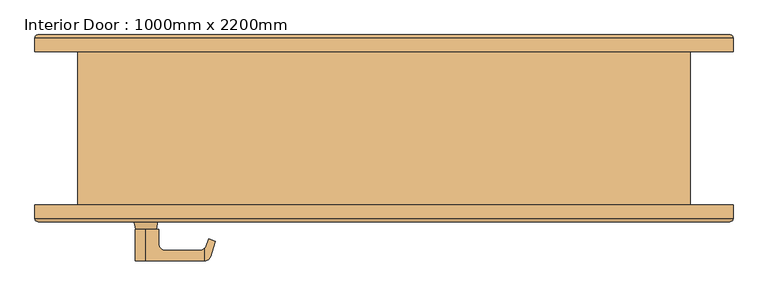
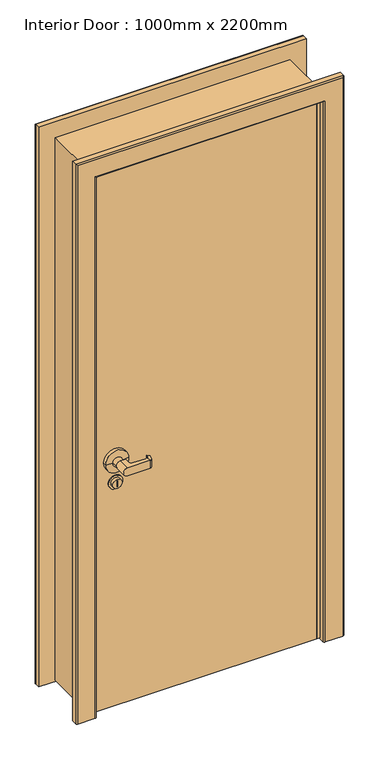
"""IFC4 building model written with IfcOpenShell, lengths in millimetres: door geometry, Interior Door : 1000mm x 2200mm."""

from ifc_helpers import new_model, si_unit, frame, origin, place, context, project, spatial, polyline, circle_curve, ellipse_curve, outline, extrude, faceted_brep, source, transform, mapped, element, save
from ifc_brep_helpers import plane_surface, cylinder_surface, revolved_surface, advanced_brep


def interior_door_1000mm_x_2200mm_056b102d(model_context):
    return source(origin(), model_context, "Body", "SolidModel", [
        advanced_brep(
        [(-323.0, -55.325, 910.0), (-377.0, -55.325, 910.0), (-368.0, -55.325, 910.0), (-332.0, -55.325, 910.0), (-349.5, -55.325, 922.0), (-349.5, -55.325, 898.0), (-350.5, -55.325, 898.0), (-350.5, -55.325, 922.0), (-323.0, -58.5, 910.0), (-377.0, -58.5, 910.0), (-332.0, -43.9713587, 910.0), (-368.0, -43.9713587, 910.0), (-349.5, -43.9713587, 898.0), (-349.5, -43.9713587, 922.0), (-350.5, -43.9713587, 922.0), (-350.5, -43.9713587, 898.0)],
        [
            (0, 1, circle_curve(frame((-350.0, -55.325, 910.0), z_axis=(0.0, 1.0, 0.0), x_axis=(-1.0, 0.0, 0.0)), 27.0)),
            (1, 0, circle_curve(frame((-350.0, -55.325, 910.0), z_axis=(0.0, 1.0, 0.0), x_axis=(-1.0, 0.0, 0.0)), 27.0)),
            (2, 3, circle_curve(frame((-350.0, -55.325, 910.0), z_axis=(0.0, -1.0, 0.0), x_axis=(-1.0, 0.0, 0.0)), 18.0)),
            (3, 2, circle_curve(frame((-350.0, -55.325, 910.0), z_axis=(0.0, -1.0, 0.0), x_axis=(-1.0, 0.0, 0.0)), 18.0)),
            (4, 5),
            (5, 6),
            (6, 7),
            (7, 4),
            (8, 9, circle_curve(frame((-350.0, -58.5, 910.0), z_axis=(0.0, -1.0, 0.0), x_axis=(-1.0, 0.0, 0.0)), 27.0)),
            (9, 8, circle_curve(frame((-350.0, -58.5, 910.0), z_axis=(0.0, -1.0, 0.0), x_axis=(-1.0, 0.0, 0.0)), 27.0)),
            (0, 8),
            (9, 1),
            (10, 11, circle_curve(frame((-350.0, -43.9713587, 910.0), z_axis=(0.0, 1.0, 0.0), x_axis=(-1.0, 0.0, 0.0)), 18.0)),
            (11, 10, circle_curve(frame((-350.0, -43.9713587, 910.0), z_axis=(0.0, 1.0, 0.0), x_axis=(-1.0, 0.0, 0.0)), 18.0)),
            (12, 13),
            (13, 14),
            (14, 15),
            (15, 12),
            (10, 3),
            (2, 11),
            (12, 5),
            (4, 13),
            (7, 14),
            (6, 15),
        ],
        [
            plane_surface(frame((-377.0, -55.325, 910.0), z_axis=(0.0, 1.0, 0.0), x_axis=(0.0, 0.0, 1.0))),
            plane_surface(frame((-377.0, -58.5, 910.0), z_axis=(0.0, -1.0, 0.0), x_axis=(0.0, 0.0, -1.0))),
            cylinder_surface(frame((-350.0, -58.5, 910.0), z_axis=(0.0, 1.0, 0.0), x_axis=(-1.0, 0.0, 0.0)), 27.0),
            plane_surface(frame((-368.0, -43.9713587, 910.0), z_axis=(0.0, 1.0, 0.0), x_axis=(0.0, 0.0, 1.0))),
            cylinder_surface(frame((-350.0, -58.5, 910.0), z_axis=(0.0, 1.0, 0.0), x_axis=(-1.0, 0.0, 0.0)), 18.0),
            plane_surface(frame((-349.5, -43.9713587, 898.0), z_axis=(-1.0, 0.0, 0.0), x_axis=(0.0, -1.0, 0.0))),
            plane_surface(frame((-349.5, -43.9713587, 922.0), z_axis=(0.0, 0.0, -1.0), x_axis=(0.0, -1.0, 0.0))),
            plane_surface(frame((-350.5, -43.9713587, 922.0), z_axis=(1.0, 0.0, 0.0), x_axis=(0.0, -1.0, 0.0))),
            plane_surface(frame((-350.5, -43.9713587, 898.0), z_axis=(0.0, 0.0, 1.0), x_axis=(0.0, -1.0, 0.0))),
        ],
        [
            (0, [[1, 2], [3, 4]]),
            (0, [[5, 6, 7, 8]]),
            (1, [[9, 10]]),
            (2, [[-1, 11, -10, 12]]),
            (2, [[-2, -12, -9, -11]]),
            (3, [[13, 14], [15, 16, 17, 18]]),
            (4, [[-13, 19, -3, 20]]),
            (4, [[-14, -20, -4, -19]]),
            (5, [[-15, 21, -5, 22]]),
            (6, [[-16, -22, -8, 23]]),
            (7, [[-17, -23, -7, 24]]),
            (8, [[-18, -24, -6, -21]]),
        ],
    ),
        advanced_brep(
        [(-323.0, -115.675, 910.0), (-377.0, -115.675, 910.0), (-368.0, -115.675, 910.0), (-332.0, -115.675, 910.0), (-349.5, -115.675, 922.0), (-350.5, -115.675, 922.0), (-350.5, -115.675, 898.0), (-349.5, -115.675, 898.0), (-323.0, -112.5, 910.0), (-377.0, -112.5, 910.0), (-332.0, -127.0286413, 910.0), (-368.0, -127.0286413, 910.0), (-349.5, -127.0286413, 898.0), (-350.5, -127.0286413, 898.0), (-350.5, -127.0286413, 922.0), (-349.5, -127.0286413, 922.0)],
        [
            (0, 1, circle_curve(frame((-350.0, -115.675, 910.0), z_axis=(0.0, -1.0, 0.0), x_axis=(-1.0, 0.0, 0.0)), 27.0)),
            (1, 0, circle_curve(frame((-350.0, -115.675, 910.0), z_axis=(0.0, -1.0, 0.0), x_axis=(-1.0, 0.0, 0.0)), 27.0)),
            (2, 3, circle_curve(frame((-350.0, -115.675, 910.0), z_axis=(0.0, 1.0, 0.0), x_axis=(-1.0, 0.0, 0.0)), 18.0)),
            (3, 2, circle_curve(frame((-350.0, -115.675, 910.0), z_axis=(0.0, 1.0, 0.0), x_axis=(-1.0, 0.0, 0.0)), 18.0)),
            (4, 5),
            (5, 6),
            (6, 7),
            (7, 4),
            (8, 9, circle_curve(frame((-350.0, -112.5, 910.0), z_axis=(0.0, 1.0, 0.0), x_axis=(-1.0, 0.0, 0.0)), 27.0)),
            (9, 8, circle_curve(frame((-350.0, -112.5, 910.0), z_axis=(0.0, 1.0, 0.0), x_axis=(-1.0, 0.0, 0.0)), 27.0)),
            (1, 9),
            (8, 0),
            (10, 11, circle_curve(frame((-350.0, -127.0286413, 910.0), z_axis=(0.0, -1.0, 0.0), x_axis=(-1.0, 0.0, 0.0)), 18.0)),
            (11, 10, circle_curve(frame((-350.0, -127.0286413, 910.0), z_axis=(0.0, -1.0, 0.0), x_axis=(-1.0, 0.0, 0.0)), 18.0)),
            (12, 13),
            (13, 14),
            (14, 15),
            (15, 12),
            (11, 2),
            (3, 10),
            (15, 4),
            (7, 12),
            (14, 5),
            (13, 6),
        ],
        [
            plane_surface(frame((-377.0, -115.675, 910.0), z_axis=(0.0, -1.0, 0.0), x_axis=(0.0, 0.0, 1.0))),
            plane_surface(frame((-377.0, -112.5, 910.0), z_axis=(0.0, 1.0, 0.0), x_axis=(0.0, 0.0, -1.0))),
            cylinder_surface(frame((-350.0, -112.5, 910.0), z_axis=(0.0, -1.0, 0.0), x_axis=(-1.0, 0.0, 0.0)), 27.0),
            plane_surface(frame((-368.0, -127.0286413, 910.0), z_axis=(0.0, -1.0, 0.0), x_axis=(0.0, 0.0, 1.0))),
            cylinder_surface(frame((-350.0, -112.5, 910.0), z_axis=(0.0, -1.0, 0.0), x_axis=(-1.0, 0.0, 0.0)), 18.0),
            plane_surface(frame((-349.5, -127.0286413, 898.0), z_axis=(-1.0, 0.0, 0.0), x_axis=(0.0, 1.0, 0.0))),
            plane_surface(frame((-349.5, -127.0286413, 922.0), z_axis=(0.0, 0.0, -1.0), x_axis=(0.0, 1.0, 0.0))),
            plane_surface(frame((-350.5, -127.0286413, 922.0), z_axis=(1.0, 0.0, 0.0), x_axis=(0.0, 1.0, 0.0))),
            plane_surface(frame((-350.5, -127.0286413, 898.0), z_axis=(0.0, 0.0, 1.0), x_axis=(0.0, 1.0, 0.0))),
        ],
        [
            (0, [[1, 2], [3, 4]]),
            (0, [[5, 6, 7, 8]]),
            (1, [[9, 10]]),
            (2, [[11, -9, 12, -2]]),
            (2, [[-12, -10, -11, -1]]),
            (3, [[13, 14], [15, 16, 17, 18]]),
            (4, [[19, -4, 20, -14]]),
            (4, [[-20, -3, -19, -13]]),
            (5, [[21, -8, 22, -18]]),
            (6, [[23, -5, -21, -17]]),
            (7, [[24, -6, -23, -16]]),
            (8, [[-22, -7, -24, -15]]),
        ],
    ),
        advanced_brep(
        [(-305.55, -125.2, 1000.0), (-394.45, -125.2, 1000.0), (-394.45, -112.5, 1000.0), (-305.55, -112.5, 1000.0), (-330.95, -128.375, 1000.0), (-369.05, -128.375, 1000.0), (-350.0, -112.5, 1000.0), (-334.9229513, -148.8140625, 1000.0), (-365.0770487, -148.8140625, 1000.0), (-350.0, -148.8140625, 1000.0)],
        [
            (0, 1, circle_curve(frame((-350.0, -125.2, 1000.0), z_axis=(0.0, 1.0, 0.0), x_axis=(-1.0, 0.0, 0.0)), 44.45)),
            (1, 2),
            (2, 3, circle_curve(frame((-350.0, -112.5, 1000.0), z_axis=(0.0, -1.0, 0.0), x_axis=(-1.0, 0.0, 0.0)), 44.45)),
            (3, 0),
            (1, 0, circle_curve(frame((-350.0, -125.2, 1000.0), z_axis=(0.0, 1.0, 0.0), x_axis=(-1.0, 0.0, 0.0)), 44.45)),
            (3, 2, circle_curve(frame((-350.0, -112.5, 1000.0), z_axis=(0.0, -1.0, 0.0), x_axis=(-1.0, 0.0, 0.0)), 44.45)),
            (4, 5, circle_curve(frame((-350.0, -128.375, 1000.0), z_axis=(0.0, 1.0, 0.0), x_axis=(-1.0, 0.0, 0.0)), 19.05)),
            (5, 1),
            (0, 4),
            (5, 4, circle_curve(frame((-350.0, -128.375, 1000.0), z_axis=(0.0, 1.0, 0.0), x_axis=(-1.0, 0.0, 0.0)), 19.05)),
            (2, 6),
            (6, 3),
            (7, 8, circle_curve(frame((-350.0, -148.8140625, 1000.0), z_axis=(0.0, 1.0, 0.0), x_axis=(-1.0, 0.0, 0.0)), 15.0770487)),
            (8, 5),
            (4, 7),
            (8, 7, circle_curve(frame((-350.0, -148.8140625, 1000.0), z_axis=(0.0, 1.0, 0.0), x_axis=(-1.0, 0.0, 0.0)), 15.0770487)),
            (9, 8),
            (7, 9),
        ],
        [
            cylinder_surface(frame((-350.0, 39.9, 1000.0), z_axis=(0.0, -1.0, 0.0), x_axis=(-1.0, 0.0, 0.0)), 44.45),
            revolved_surface(polyline([(-394.45, -125.2, 1000.0), (-369.05, -128.375, 1000.0)]), (-350.0, 39.9, 1000.0), (0.0, -1.0, 0.0)),
            plane_surface(frame((-350.0, -112.5, 1000.0), z_axis=(0.0, 1.0, 0.0), x_axis=(-1.0, 0.0, 0.0))),
            revolved_surface(polyline([(-369.05, -128.375, 1000.0), (-365.0770487, -148.8140625, 1000.0)]), (-350.0, 39.9, 1000.0), (0.0, -1.0, 0.0)),
            plane_surface(frame((-350.0, -148.8140625, 1000.0), z_axis=(0.0, -1.0, 0.0), x_axis=(-1.0, 0.0, 0.0))),
        ],
        [
            (0, [[1, 2, 3, 4]]),
            (0, [[5, -4, 6, -2]]),
            (1, [[7, 8, -1, 9]]),
            (1, [[10, -9, -5, -8]]),
            (2, [[-3, 11, 12]]),
            (2, [[-6, -12, -11]]),
            (3, [[13, 14, -7, 15]]),
            (3, [[16, -15, -10, -14]]),
            (4, [[17, -13, 18]]),
            (4, [[-18, -16, -17]]),
        ],
    ),
        advanced_brep(
        [(-330.95, -169.7736937, 1015.875), (-330.95, -148.8140625, 1015.875), (-350.0, -148.8140625, 1015.875), (-350.0, -195.05, 1015.875), (-264.0071516, -195.05, 1015.875), (-264.0071516, -176.7564308, 1015.875), (-270.4853465, -179.2986937, 1015.875), (-321.425, -179.2986937, 1015.875), (-330.95, -169.7736937, 984.125), (-321.425, -179.2986937, 984.125), (-270.4853465, -179.2986937, 984.125), (-264.0071516, -176.7564308, 984.125), (-264.0071516, -195.05, 984.125), (-350.0, -195.05, 984.125), (-350.0, -148.8140625, 984.125), (-330.95, -148.8140625, 984.125), (-261.5347742, -173.0314356, 1015.2888063), (-261.5347742, -173.0314356, 984.7111937), (-257.8148231, -162.8109537, 1014.4068164), (-257.8148231, -162.8109537, 985.5931836), (-247.6815328, -166.1034593, 1012.0042419), (-247.6815328, -166.1034593, 987.9957581), (-254.9483383, -188.4683869, 1013.727181), (-254.9483383, -188.4683869, 986.272819)],
        [
            (0, 1),
            (1, 2),
            (2, 3),
            (3, 4),
            (4, 5),
            (5, 6, circle_curve(frame((-270.4853465, -169.7736937, 1015.875), z_axis=(0.0, 0.0, -1.0), x_axis=(1.0, 0.0, 0.0)), 9.525)),
            (6, 7),
            (7, 0, circle_curve(frame((-321.425, -169.7736937, 1015.875), z_axis=(0.0, 0.0, -1.0), x_axis=(1.0, 0.0, 0.0)), 9.525)),
            (8, 9, circle_curve(frame((-321.425, -169.7736937, 984.125), z_axis=(0.0, 0.0, 1.0), x_axis=(1.0, 0.0, 0.0)), 9.525)),
            (9, 10),
            (10, 11, circle_curve(frame((-270.4853465, -169.7736937, 984.125), z_axis=(0.0, 0.0, 1.0), x_axis=(1.0, 0.0, 0.0)), 9.525)),
            (11, 12),
            (12, 13),
            (13, 14),
            (14, 15),
            (15, 8),
            (0, 8),
            (15, 1),
            (6, 10),
            (9, 7),
            (12, 4),
            (3, 13, circle_curve(frame((-350.0, -195.05, 1000.0), z_axis=(0.0, -1.0, 0.0), x_axis=(0.0, 0.0, 1.0)), 15.875)),
            (14, 2, circle_curve(frame((-350.0, -148.8140625, 1000.0), z_axis=(0.0, 1.0, 0.0), x_axis=(0.0, 0.0, 1.0)), 15.875)),
            (5, 16, ellipse_curve(frame((-270.4853465, -169.7736937, 1017.4109617), z_axis=(0.23070138294863687, 0.0, 0.9730245998460607), x_axis=(-0.9730245998460608, 0.0, 0.23070138294863632)), 9.7890639, 9.525)),
            (16, 17),
            (17, 11, ellipse_curve(frame((-270.4853465, -169.7736937, 982.5890383), z_axis=(0.23070138294863055, 0.0, -0.9730245998460623), x_axis=(0.9730245998460625, 0.0, 0.23070138294862935)), 9.7890639, 9.525)),
            (16, 18),
            (18, 19),
            (19, 17),
            (18, 20),
            (20, 21),
            (21, 19),
            (20, 22),
            (22, 23),
            (23, 21),
            (12, 23, ellipse_curve(frame((-264.0071516, -185.525, 984.125), z_axis=(-0.23070138294863055, 0.0, 0.9730245998460623), x_axis=(-0.9730245998460625, 0.0, -0.23070138294862935)), 9.7890639, 9.525)),
            (22, 4, ellipse_curve(frame((-264.0071516, -185.525, 1015.875), z_axis=(-0.23070138294863687, 0.0, -0.9730245998460607), x_axis=(0.9730245998460608, 0.0, -0.23070138294863632)), 9.7890639, 9.525)),
        ],
        [
            plane_surface(frame((-311.9, -169.7736937, 1015.875), z_axis=(0.0, 0.0, 1.0), x_axis=(0.0, -1.0, 0.0))),
            plane_surface(frame((-311.9, -169.7736937, 984.125), z_axis=(0.0, 0.0, -1.0), x_axis=(0.0, 1.0, 0.0))),
            plane_surface(frame((-330.95, -148.8140625, 984.125), z_axis=(1.0, 0.0, 0.0), x_axis=(0.0, 0.0, 1.0))),
            plane_surface(frame((-321.425, -179.2986937, 984.125), z_axis=(0.0, 1.0, 0.0), x_axis=(0.0, 0.0, 1.0))),
            plane_surface(frame((-264.0071516, -195.05, 984.125), z_axis=(0.0, -1.0, 0.0), x_axis=(0.0, 0.0, 1.0))),
            plane_surface(frame((-369.05, -148.8140625, 984.125), z_axis=(0.0, 1.0, 0.0), x_axis=(0.0, 0.0, 1.0))),
            revolved_surface(polyline([(-311.90000000000003, -169.7736937, 1015.875), (-311.90000000000003, -169.7736937, 984.125)]), (-321.425, -169.7736937, 1015.875), (0.0, 0.0, 1.0)),
            revolved_surface(polyline([(-260.9603465, -169.7736937, 1019.6693122795026), (-260.9603465, -169.7736937, 980.3306877204975)]), (-270.4853465, -169.7736937, 1015.875), (0.0, 0.0, 1.0)),
            plane_surface(frame((-261.5347742, -173.0314356, 984.125), z_axis=(-0.93969262078591, 0.3420201433256644, 0.0), x_axis=(0.0, 0.0, 1.0))),
            plane_surface(frame((-257.8148231, -162.8109537, 984.125), z_axis=(0.30901699437494523, 0.9510565162951543, 0.0), x_axis=(0.0, 0.0, 1.0))),
            plane_surface(frame((-247.6815328, -166.1034593, 984.125), z_axis=(0.9510565162951542, -0.3090169943749457, 0.0), x_axis=(0.0, 0.0, 1.0))),
            cylinder_surface(frame((-264.0071516, -185.525, 1015.875), z_axis=(0.0, 0.0, -1.0), x_axis=(1.0, 0.0, 0.0)), 9.525),
            cylinder_surface(frame((-350.0, -417.3, 1000.0), z_axis=(0.0, -1.0, 0.0), x_axis=(0.0, 0.0, 1.0)), 15.875),
            plane_surface(frame((-264.0071516, 192.3, 984.125), z_axis=(0.23070138294863055, 0.0, -0.9730245998460623), x_axis=(0.0, -1.0, 0.0))),
            plane_surface(frame((-236.70001, 192.3, 1009.4005539), z_axis=(0.23070138294863687, 0.0, 0.9730245998460607), x_axis=(0.0, -1.0, 0.0))),
        ],
        [
            (0, [[1, 2, 3, 4, 5, 6, 7, 8]]),
            (1, [[9, 10, 11, 12, 13, 14, 15, 16]]),
            (2, [[-1, 17, -16, 18]]),
            (3, [[-7, 19, -10, 20]]),
            (4, [[21, -4, 22, -13]]),
            (5, [[-18, -15, 23, -2]]),
            (6, [[-8, -20, -9, -17]]),
            (7, [[-19, -6, 24, 25, 26, -11]]),
            (8, [[-25, 27, 28, 29]]),
            (9, [[-28, 30, 31, 32]]),
            (10, [[-31, 33, 34, 35]]),
            (11, [[-21, 36, -34, 37]]),
            (12, [[-3, -23, -14, -22]]),
            (13, [[-12, -26, -29, -32, -35, -36]]),
            (14, [[-5, -37, -33, -30, -27, -24]]),
        ],
    ),
        advanced_brep(
        [(-305.55, -45.8, 1000.0), (-305.55, -58.5, 1000.0), (-394.45, -58.5, 1000.0), (-394.45, -45.8, 1000.0), (-330.95, -42.625, 1000.0), (-369.05, -42.625, 1000.0), (-350.0, -58.5, 1000.0), (-334.9229513, -22.1859375, 1000.0), (-365.0770487, -22.1859375, 1000.0), (-350.0, -22.1859375, 1000.0)],
        [
            (0, 1),
            (1, 2, circle_curve(frame((-350.0, -58.5, 1000.0), z_axis=(0.0, 1.0, 0.0), x_axis=(-1.0, 0.0, 0.0)), 44.45)),
            (2, 3),
            (3, 0, circle_curve(frame((-350.0, -45.8, 1000.0), z_axis=(0.0, -1.0, 0.0), x_axis=(-1.0, 0.0, 0.0)), 44.45)),
            (2, 1, circle_curve(frame((-350.0, -58.5, 1000.0), z_axis=(0.0, 1.0, 0.0), x_axis=(-1.0, 0.0, 0.0)), 44.45)),
            (0, 3, circle_curve(frame((-350.0, -45.8, 1000.0), z_axis=(0.0, -1.0, 0.0), x_axis=(-1.0, 0.0, 0.0)), 44.45)),
            (4, 0),
            (3, 5),
            (5, 4, circle_curve(frame((-350.0, -42.625, 1000.0), z_axis=(0.0, -1.0, 0.0), x_axis=(-1.0, 0.0, 0.0)), 19.05)),
            (4, 5, circle_curve(frame((-350.0, -42.625, 1000.0), z_axis=(0.0, -1.0, 0.0), x_axis=(-1.0, 0.0, 0.0)), 19.05)),
            (1, 6),
            (6, 2),
            (7, 4),
            (5, 8),
            (8, 7, circle_curve(frame((-350.0, -22.1859375, 1000.0), z_axis=(0.0, -1.0, 0.0), x_axis=(-1.0, 0.0, 0.0)), 15.0770487)),
            (7, 8, circle_curve(frame((-350.0, -22.1859375, 1000.0), z_axis=(0.0, -1.0, 0.0), x_axis=(-1.0, 0.0, 0.0)), 15.0770487)),
            (9, 7),
            (8, 9),
        ],
        [
            cylinder_surface(frame((-350.0, -210.9, 1000.0), z_axis=(0.0, 1.0, 0.0), x_axis=(-1.0, 0.0, 0.0)), 44.45),
            revolved_surface(polyline([(-394.45, -45.8, 1000.0), (-369.05, -42.625, 1000.0)]), (-350.0, -210.9, 1000.0), (0.0, 1.0, 0.0)),
            plane_surface(frame((-350.0, -58.5, 1000.0), z_axis=(0.0, -1.0, 0.0), x_axis=(-1.0, 0.0, 0.0))),
            revolved_surface(polyline([(-369.05, -42.625, 1000.0), (-365.0770487, -22.1859375, 1000.0)]), (-350.0, -210.9, 1000.0), (0.0, 1.0, 0.0)),
            plane_surface(frame((-350.0, -22.1859375, 1000.0), z_axis=(0.0, 1.0, 0.0), x_axis=(-1.0, 0.0, 0.0))),
        ],
        [
            (0, [[1, 2, 3, 4]]),
            (0, [[-3, 5, -1, 6]]),
            (1, [[7, -4, 8, 9]]),
            (1, [[-8, -6, -7, 10]]),
            (2, [[11, 12, -2]]),
            (2, [[-12, -11, -5]]),
            (3, [[13, -9, 14, 15]]),
            (3, [[-14, -10, -13, 16]]),
            (4, [[17, -15, 18]]),
            (4, [[-18, -16, -17]]),
        ],
    ),
        advanced_brep(
        [(-330.95, -1.2263063, 1015.875), (-321.425, 8.2986937, 1015.875), (-270.4853465, 8.2986937, 1015.875), (-264.0071516, 5.7564308, 1015.875), (-264.0071516, 24.05, 1015.875), (-350.0, 24.05, 1015.875), (-350.0, -22.1859375, 1015.875), (-330.95, -22.1859375, 1015.875), (-330.95, -1.2263063, 984.125), (-330.95, -22.1859375, 984.125), (-350.0, -22.1859375, 984.125), (-350.0, 24.05, 984.125), (-264.0071516, 24.05, 984.125), (-264.0071516, 5.7564308, 984.125), (-270.4853465, 8.2986937, 984.125), (-321.425, 8.2986937, 984.125), (-261.5347742, 2.0314356, 984.7111937), (-261.5347742, 2.0314356, 1015.2888063), (-257.8148231, -8.1890463, 985.5931836), (-257.8148231, -8.1890463, 1014.4068164), (-247.6815328, -4.8965407, 987.9957581), (-247.6815328, -4.8965407, 1012.0042419), (-254.9483383, 17.4683869, 986.272819), (-254.9483383, 17.4683869, 1013.727181)],
        [
            (0, 1, circle_curve(frame((-321.425, -1.2263063, 1015.875), z_axis=(0.0, 0.0, -1.0), x_axis=(1.0, 0.0, 0.0)), 9.525)),
            (1, 2),
            (2, 3, circle_curve(frame((-270.4853465, -1.2263063, 1015.875), z_axis=(0.0, 0.0, -1.0), x_axis=(1.0, 0.0, 0.0)), 9.525)),
            (3, 4),
            (4, 5),
            (5, 6),
            (6, 7),
            (7, 0),
            (8, 9),
            (9, 10),
            (10, 11),
            (11, 12),
            (12, 13),
            (13, 14, circle_curve(frame((-270.4853465, -1.2263063, 984.125), z_axis=(0.0, 0.0, 1.0), x_axis=(1.0, 0.0, 0.0)), 9.525)),
            (14, 15),
            (15, 8, circle_curve(frame((-321.425, -1.2263063, 984.125), z_axis=(0.0, 0.0, 1.0), x_axis=(1.0, 0.0, 0.0)), 9.525)),
            (7, 9),
            (8, 0),
            (1, 15),
            (14, 2),
            (11, 5, circle_curve(frame((-350.0, 24.05, 1000.0), z_axis=(0.0, 1.0, 0.0), x_axis=(0.0, 0.0, 1.0)), 15.875)),
            (4, 12),
            (6, 10, circle_curve(frame((-350.0, -22.1859375, 1000.0), z_axis=(0.0, -1.0, 0.0), x_axis=(0.0, 0.0, 1.0)), 15.875)),
            (13, 16, ellipse_curve(frame((-270.4853465, -1.2263063, 982.5890383), z_axis=(0.23070138294863055, 0.0, -0.9730245998460623), x_axis=(0.9730245998460625, 0.0, 0.23070138294862935)), 9.7890639, 9.525)),
            (16, 17),
            (17, 3, ellipse_curve(frame((-270.4853465, -1.2263063, 1017.4109617), z_axis=(0.23070138294863687, 0.0, 0.9730245998460607), x_axis=(-0.9730245998460608, 0.0, 0.23070138294863632)), 9.7890639, 9.525)),
            (16, 18),
            (18, 19),
            (19, 17),
            (18, 20),
            (20, 21),
            (21, 19),
            (20, 22),
            (22, 23),
            (23, 21),
            (4, 23, ellipse_curve(frame((-264.0071516, 14.525, 1015.875), z_axis=(-0.23070138294863687, 0.0, -0.9730245998460607), x_axis=(0.9730245998460608, 0.0, -0.23070138294863632)), 9.7890639, 9.525)),
            (22, 12, ellipse_curve(frame((-264.0071516, 14.525, 984.125), z_axis=(-0.23070138294863055, 0.0, 0.9730245998460623), x_axis=(-0.9730245998460625, 0.0, -0.23070138294862935)), 9.7890639, 9.525)),
        ],
        [
            plane_surface(frame((-311.9, -1.2263063, 1015.875), z_axis=(0.0, 0.0, 1.0), x_axis=(0.0, 1.0, 0.0))),
            plane_surface(frame((-311.9, -1.2263063, 984.125), z_axis=(0.0, 0.0, -1.0), x_axis=(0.0, -1.0, 0.0))),
            plane_surface(frame((-330.95, -22.1859375, 984.125), z_axis=(1.0, 0.0, 0.0), x_axis=(0.0, 0.0, 1.0))),
            plane_surface(frame((-321.425, 8.2986937, 984.125), z_axis=(0.0, -1.0, 0.0), x_axis=(0.0, 0.0, 1.0))),
            plane_surface(frame((-264.0071516, 24.05, 984.125), z_axis=(0.0, 1.0, 0.0), x_axis=(0.0, 0.0, 1.0))),
            plane_surface(frame((-369.05, -22.1859375, 984.125), z_axis=(0.0, -1.0, 0.0), x_axis=(0.0, 0.0, 1.0))),
            revolved_surface(polyline([(-311.90000000000003, -1.2263063, 1015.875), (-311.90000000000003, -1.2263063, 984.125)]), (-321.425, -1.2263063, 1015.875), (0.0, 0.0, 1.0)),
            revolved_surface(polyline([(-260.9603465, -1.2263063, 1019.6693122795026), (-260.9603465, -1.2263063, 980.3306877204975)]), (-270.4853465, -1.2263063, 1015.875), (0.0, 0.0, 1.0)),
            plane_surface(frame((-261.5347742, 2.0314356, 984.125), z_axis=(-0.93969262078591, -0.3420201433256644, 0.0), x_axis=(0.0, 0.0, 1.0))),
            plane_surface(frame((-257.8148231, -8.1890463, 984.125), z_axis=(0.30901699437494523, -0.9510565162951543, 0.0), x_axis=(0.0, 0.0, 1.0))),
            plane_surface(frame((-247.6815328, -4.8965407, 984.125), z_axis=(0.9510565162951542, 0.3090169943749457, 0.0), x_axis=(0.0, 0.0, 1.0))),
            cylinder_surface(frame((-264.0071516, 14.525, 1015.875), z_axis=(0.0, 0.0, -1.0), x_axis=(1.0, 0.0, 0.0)), 9.525),
            cylinder_surface(frame((-350.0, 246.3, 1000.0), z_axis=(0.0, 1.0, 0.0), x_axis=(0.0, 0.0, 1.0)), 15.875),
            plane_surface(frame((-264.0071516, -363.3, 984.125), z_axis=(0.23070138294863055, 0.0, -0.9730245998460623), x_axis=(0.0, 1.0, 0.0))),
            plane_surface(frame((-236.70001, -363.3, 1009.4005539), z_axis=(0.23070138294863687, 0.0, 0.9730245998460607), x_axis=(0.0, 1.0, 0.0))),
        ],
        [
            (0, [[1, 2, 3, 4, 5, 6, 7, 8]]),
            (1, [[9, 10, 11, 12, 13, 14, 15, 16]]),
            (2, [[17, -9, 18, -8]]),
            (3, [[19, -15, 20, -2]]),
            (4, [[-12, 21, -5, 22]]),
            (5, [[-7, 23, -10, -17]]),
            (6, [[-18, -16, -19, -1]]),
            (7, [[-14, 24, 25, 26, -3, -20]]),
            (8, [[27, 28, 29, -25]]),
            (9, [[30, 31, 32, -28]]),
            (10, [[33, 34, 35, -31]]),
            (11, [[36, -34, 37, -22]]),
            (12, [[-21, -11, -23, -6]]),
            (13, [[-37, -33, -30, -27, -24, -13]]),
            (14, [[-26, -29, -32, -35, -36, -4]]),
        ],
    ),
        extrude(outline(polyline([(422.0000374, -58.5), (422.0000374, -112.5), (-422.0000374, -112.5), (-422.0000374, -58.5), (422.0000374, -58.5)])), frame((0.0, 0.0, 5.0), z_axis=(0.0, 0.0, 1.0), x_axis=(1.0, 0.0, 0.0)), (0.0, 0.0, 1.0), 2167.0000374),
        faceted_brep([(-405.0000128, -58.5, 5.0), (-422.0000374, -58.5, 5.0), (-422.0000374, -112.5, 5.0), (-450.0, -112.5, 5.0), (-450.0, 112.5, 5.0), (-405.0000128, 112.5, 5.0), (-405.0000128, 112.5, 2155.0000128), (-405.0000128, -58.5, 2155.0000128), (-450.0, 112.5, 2200.0), (450.0, 112.5, 2200.0), (450.0, 112.5, 5.0), (405.0000128, 112.5, 5.0), (405.0000128, 112.5, 2155.0000128), (-450.0, -112.5, 2200.0), (-422.0000374, -112.5, 2172.0000374), (422.0000374, -112.5, 2172.0000374), (422.0000374, -112.5, 5.0), (450.0, -112.5, 5.0), (450.0, -112.5, 2200.0), (-422.0000374, -58.5, 2172.0000374), (405.0000128, -58.5, 2155.0000128), (405.0000128, -58.5, 5.0), (422.0000374, -58.5, 5.0), (422.0000374, -58.5, 2172.0000374)], [[[0, 1, 2, 3, 4, 5]], [[0, 5, 6, 7]], [[4, 8, 9, 10, 11, 12, 6, 5]], [[3, 13, 8, 4]], [[2, 14, 15, 16, 17, 18, 13, 3]], [[1, 19, 14, 2]], [[0, 7, 20, 21, 22, 23, 19, 1]], [[12, 11, 21, 20]], [[11, 10, 17, 16, 22, 21]], [[18, 17, 10, 9]], [[23, 22, 16, 15]], [[13, 18, 9, 8]], [[19, 23, 15, 14]], [[6, 12, 20, 7]]]),
        advanced_brep(
        [(-439.9983436, -137.5, 0.0), (-507.9986597, -137.5, 0.0), (-512.9993919, -132.4992678, 0.0), (-512.9993919, -112.5, 0.0), (-435.0, -112.5, 0.0), (-435.0, -132.5016564, 0.0), (-435.0, -132.5016564, 2185.0), (-439.9983436, -137.5, 2189.9983436), (-435.0, -112.5, 2185.0), (-512.9993919, -112.5, 2262.9993919), (512.9993919, -112.5, 2262.9993919), (512.9993919, -112.5, 0.0), (435.0, -112.5, 0.0), (435.0, -112.5, 2185.0), (-512.9993919, -132.4992678, 2262.9993919), (-507.9986597, -137.5, 2257.9986597), (439.9983436, -137.5, 2189.9983436), (439.9983436, -137.5, 0.0), (507.9986597, -137.5, 0.0), (507.9986597, -137.5, 2257.9986597), (435.0, -132.5016564, 0.0), (435.0, -132.5016564, 2185.0), (512.9993919, -132.4992678, 0.0), (512.9993919, -132.4992678, 2262.9993919)],
        [
            (0, 1),
            (1, 2, circle_curve(frame((-507.9986597, -132.4992678, 0.0), z_axis=(0.0, 0.0, -1.0), x_axis=(-1.0, 0.0, 0.0)), 5.0007322)),
            (2, 3),
            (3, 4),
            (4, 5),
            (5, 0, circle_curve(frame((-439.9983436, -132.5016564, 0.0), z_axis=(0.0, 0.0, -1.0), x_axis=(-1.0, 0.0, 0.0)), 4.9983436)),
            (5, 6),
            (6, 7, ellipse_curve(frame((-439.9983436, -132.5016564, 2189.9983436), z_axis=(-0.7071067811865475, 0.0, -0.7071067811865475), x_axis=(0.7071067811865474, 0.0, -0.7071067811865476)), 7.0687253, 4.9983436)),
            (7, 0),
            (4, 8),
            (8, 6),
            (3, 9),
            (9, 10),
            (10, 11),
            (11, 12),
            (12, 13),
            (13, 8),
            (2, 14),
            (14, 9),
            (1, 15),
            (15, 14, ellipse_curve(frame((-507.9986597, -132.4992678, 2257.9986597), z_axis=(-0.7071067811865475, 0.0, -0.7071067811865475), x_axis=(0.7071067811865474, 0.0, -0.7071067811865476)), 7.0721032, 5.0007322)),
            (7, 16),
            (16, 17),
            (17, 18),
            (18, 19),
            (19, 15),
            (12, 20),
            (20, 21),
            (21, 13),
            (17, 20, circle_curve(frame((439.9983436, -132.5016564, 0.0), z_axis=(0.0, 0.0, -1.0), x_axis=(1.0, 0.0, 0.0)), 4.9983436)),
            (11, 22),
            (22, 18, circle_curve(frame((507.9986597, -132.4992678, 0.0), z_axis=(0.0, 0.0, -1.0), x_axis=(1.0, 0.0, 0.0)), 5.0007322)),
            (23, 22),
            (10, 23),
            (23, 19, ellipse_curve(frame((507.9986597, -132.4992678, 2257.9986597), z_axis=(0.7071067811865475, 0.0, -0.7071067811865475), x_axis=(0.7071067811865474, 0.0, 0.7071067811865476)), 7.0721032, 5.0007322)),
            (16, 21, ellipse_curve(frame((439.9983436, -132.5016564, 2189.9983436), z_axis=(0.7071067811865475, 0.0, -0.7071067811865475), x_axis=(0.7071067811865474, 0.0, 0.7071067811865476)), 7.0687253, 4.9983436)),
            (6, 21),
            (14, 23),
        ],
        [
            plane_surface(frame((-450.0, 125.0, 0.0), z_axis=(0.0, 0.0, -1.0), x_axis=(0.0, 1.0, 0.0))),
            cylinder_surface(frame((-439.9983436, -132.5016564, 0.0), z_axis=(0.0, 0.0, -1.0), x_axis=(-1.0, 0.0, 0.0)), 4.9983436),
            plane_surface(frame((-435.0, -132.5016564, 0.0), z_axis=(1.0, 0.0, 0.0), x_axis=(0.0, 0.0, 1.0))),
            plane_surface(frame((-435.0, -112.5, 0.0), z_axis=(0.0, 1.0, 0.0), x_axis=(0.0, 0.0, 1.0))),
            plane_surface(frame((-512.9993919, -112.5, 0.0), z_axis=(-1.0, 0.0, 0.0), x_axis=(0.0, 0.0, 1.0))),
            cylinder_surface(frame((-507.9986597, -132.4992678, 0.0), z_axis=(0.0, 0.0, -1.0), x_axis=(-1.0, 0.0, 0.0)), 5.0007322),
            plane_surface(frame((-507.9986597, -137.5, 0.0), z_axis=(0.0, -1.0, 0.0), x_axis=(0.0, 0.0, 1.0))),
            plane_surface(frame((435.0, -132.5016564, 2185.0), z_axis=(-1.0, 0.0, 0.0), x_axis=(0.0, 0.0, -1.0))),
            plane_surface(frame((450.0, 125.0, 0.0), z_axis=(0.0, 0.0, -1.0), x_axis=(0.0, 1.0, 0.0))),
            plane_surface(frame((512.9993919, -112.5, 2262.9993919), z_axis=(1.0, 0.0, 0.0), x_axis=(0.0, 0.0, -1.0))),
            cylinder_surface(frame((507.9986597, -132.4992678, 2200.0), z_axis=(0.0, 0.0, 1.0), x_axis=(1.0, 0.0, 0.0)), 5.0007322),
            cylinder_surface(frame((439.9983436, -132.5016564, 2200.0), z_axis=(0.0, 0.0, 1.0), x_axis=(1.0, 0.0, 0.0)), 4.9983436),
            cylinder_surface(frame((-450.0, -132.5016564, 2189.9983436), z_axis=(-1.0, 0.0, 0.0), x_axis=(0.0, 0.0, 1.0)), 4.9983436),
            plane_surface(frame((-435.0, -132.5016564, 2185.0), z_axis=(0.0, 0.0, -1.0), x_axis=(1.0, 0.0, 0.0))),
            plane_surface(frame((-512.9993919, -112.5, 2262.9993919), z_axis=(0.0, 0.0, 1.0), x_axis=(1.0, 0.0, 0.0))),
            cylinder_surface(frame((-450.0, -132.4992678, 2257.9986597), z_axis=(-1.0, 0.0, 0.0), x_axis=(0.0, 0.0, 1.0)), 5.0007322),
        ],
        [
            (0, [[1, 2, 3, 4, 5, 6]]),
            (1, [[7, 8, 9, -6]]),
            (2, [[10, 11, -7, -5]]),
            (3, [[12, 13, 14, 15, 16, 17, -10, -4]]),
            (4, [[18, 19, -12, -3]]),
            (5, [[20, 21, -18, -2]]),
            (6, [[-9, 22, 23, 24, 25, 26, -20, -1]]),
            (7, [[-16, 27, 28, 29]]),
            (8, [[30, -27, -15, 31, 32, -24]]),
            (9, [[33, -31, -14, 34]]),
            (10, [[-25, -32, -33, 35]]),
            (11, [[-28, -30, -23, 36]]),
            (12, [[37, -36, -22, -8]]),
            (13, [[-17, -29, -37, -11]]),
            (14, [[38, -34, -13, -19]]),
            (15, [[-26, -35, -38, -21]]),
        ],
    ),
        advanced_brep(
        [(-439.9983436, 137.5, 0.0), (-435.0, 132.5016564, 0.0), (-435.0, 112.5, 0.0), (-512.9993919, 112.5, 0.0), (-512.9993919, 132.4992678, 0.0), (-507.9986597, 137.5, 0.0), (-507.9986597, 137.5, 2257.9986597), (507.9986597, 137.5, 2257.9986597), (507.9986597, 137.5, 0.0), (439.9983436, 137.5, 0.0), (439.9983436, 137.5, 2189.9983436), (-439.9983436, 137.5, 2189.9983436), (-512.9993919, 132.4992678, 2262.9993919), (-512.9993919, 112.5, 2262.9993919), (-435.0, 112.5, 2185.0), (435.0, 112.5, 2185.0), (435.0, 112.5, 0.0), (512.9993919, 112.5, 0.0), (512.9993919, 112.5, 2262.9993919), (-435.0, 132.5016564, 2185.0), (512.9993919, 132.4992678, 0.0), (512.9993919, 132.4992678, 2262.9993919), (435.0, 132.5016564, 0.0), (435.0, 132.5016564, 2185.0)],
        [
            (0, 1, circle_curve(frame((-439.9983436, 132.5016564, 0.0), z_axis=(0.0, 0.0, -1.0), x_axis=(1.0, 0.0, 0.0)), 4.9983436)),
            (1, 2),
            (2, 3),
            (3, 4),
            (4, 5, circle_curve(frame((-507.9986597, 132.4992678, 0.0), z_axis=(0.0, 0.0, -1.0), x_axis=(1.0, 0.0, 0.0)), 5.0007322)),
            (5, 0),
            (5, 6),
            (6, 7),
            (7, 8),
            (8, 9),
            (9, 10),
            (10, 11),
            (11, 0),
            (4, 12),
            (12, 6, ellipse_curve(frame((-507.9986597, 132.4992678, 2257.9986597), z_axis=(-0.7071067811865475, 0.0, -0.7071067811865475), x_axis=(0.7071067811865474, 0.0, -0.7071067811865476)), 7.0721032, 5.0007322)),
            (3, 13),
            (13, 12),
            (2, 14),
            (14, 15),
            (15, 16),
            (16, 17),
            (17, 18),
            (18, 13),
            (1, 19),
            (19, 14),
            (11, 19, ellipse_curve(frame((-439.9983436, 132.5016564, 2189.9983436), z_axis=(-0.7071067811865475, 0.0, -0.7071067811865475), x_axis=(0.7071067811865474, 0.0, -0.7071067811865476)), 7.0687253, 4.9983436)),
            (17, 20),
            (20, 21),
            (21, 18),
            (8, 20, circle_curve(frame((507.9986597, 132.4992678, 0.0), z_axis=(0.0, 0.0, -1.0), x_axis=(-1.0, 0.0, 0.0)), 5.0007322)),
            (16, 22),
            (22, 9, circle_curve(frame((439.9983436, 132.5016564, 0.0), z_axis=(0.0, 0.0, -1.0), x_axis=(-1.0, 0.0, 0.0)), 4.9983436)),
            (23, 22),
            (15, 23),
            (23, 10, ellipse_curve(frame((439.9983436, 132.5016564, 2189.9983436), z_axis=(0.7071067811865475, 0.0, -0.7071067811865475), x_axis=(0.7071067811865474, 0.0, 0.7071067811865476)), 7.0687253, 4.9983436)),
            (7, 21, ellipse_curve(frame((507.9986597, 132.4992678, 2257.9986597), z_axis=(0.7071067811865475, 0.0, -0.7071067811865475), x_axis=(0.7071067811865474, 0.0, 0.7071067811865476)), 7.0721032, 5.0007322)),
            (23, 19),
            (21, 12),
        ],
        [
            plane_surface(frame((-450.0, -125.0, 0.0), z_axis=(0.0, 0.0, -1.0), x_axis=(0.0, -1.0, 0.0))),
            plane_surface(frame((-439.9983436, 137.5, 0.0), z_axis=(0.0, 1.0, 0.0), x_axis=(0.0, 0.0, 1.0))),
            cylinder_surface(frame((-507.9986597, 132.4992678, 0.0), z_axis=(0.0, 0.0, -1.0), x_axis=(1.0, 0.0, 0.0)), 5.0007322),
            plane_surface(frame((-512.9993919, 132.4992678, 0.0), z_axis=(-1.0, 0.0, 0.0), x_axis=(0.0, 0.0, 1.0))),
            plane_surface(frame((-512.9993919, 112.5, 0.0), z_axis=(0.0, -1.0, 0.0), x_axis=(0.0, 0.0, 1.0))),
            plane_surface(frame((-435.0, 112.5, 0.0), z_axis=(1.0, 0.0, 0.0), x_axis=(0.0, 0.0, 1.0))),
            cylinder_surface(frame((-439.9983436, 132.5016564, 0.0), z_axis=(0.0, 0.0, -1.0), x_axis=(1.0, 0.0, 0.0)), 4.9983436),
            plane_surface(frame((512.9993919, 132.4992678, 2262.9993919), z_axis=(1.0, 0.0, 0.0), x_axis=(0.0, 0.0, -1.0))),
            plane_surface(frame((450.0, -125.0, 0.0), z_axis=(0.0, 0.0, -1.0), x_axis=(0.0, -1.0, 0.0))),
            plane_surface(frame((435.0, 112.5, 2185.0), z_axis=(-1.0, 0.0, 0.0), x_axis=(0.0, 0.0, -1.0))),
            cylinder_surface(frame((439.9983436, 132.5016564, 2200.0), z_axis=(0.0, 0.0, 1.0), x_axis=(-1.0, 0.0, 0.0)), 4.9983436),
            cylinder_surface(frame((507.9986597, 132.4992678, 2200.0), z_axis=(0.0, 0.0, 1.0), x_axis=(-1.0, 0.0, 0.0)), 5.0007322),
            cylinder_surface(frame((-450.0, 132.5016564, 2189.9983436), z_axis=(-1.0, 0.0, 0.0), x_axis=(0.0, 0.0, -1.0)), 4.9983436),
            plane_surface(frame((-435.0, 112.5, 2185.0), z_axis=(0.0, 0.0, -1.0), x_axis=(1.0, 0.0, 0.0))),
            plane_surface(frame((-512.9993919, 132.4992678, 2262.9993919), z_axis=(0.0, 0.0, 1.0), x_axis=(1.0, 0.0, 0.0))),
            cylinder_surface(frame((-450.0, 132.4992678, 2257.9986597), z_axis=(-1.0, 0.0, 0.0), x_axis=(0.0, 0.0, -1.0)), 5.0007322),
        ],
        [
            (0, [[1, 2, 3, 4, 5, 6]]),
            (1, [[7, 8, 9, 10, 11, 12, 13, -6]]),
            (2, [[14, 15, -7, -5]]),
            (3, [[16, 17, -14, -4]]),
            (4, [[18, 19, 20, 21, 22, 23, -16, -3]]),
            (5, [[24, 25, -18, -2]]),
            (6, [[-13, 26, -24, -1]]),
            (7, [[-22, 27, 28, 29]]),
            (8, [[-10, 30, -27, -21, 31, 32]]),
            (9, [[33, -31, -20, 34]]),
            (10, [[-11, -32, -33, 35]]),
            (11, [[-28, -30, -9, 36]]),
            (12, [[-12, -35, 37, -26]]),
            (13, [[-37, -34, -19, -25]]),
            (14, [[-23, -29, 38, -17]]),
            (15, [[-38, -36, -8, -15]]),
        ],
    ),
    ])


if __name__ == "__main__":
    model = new_model("IFC4")
    model_context = context("Model", 3, world=origin())
    ifc_project = project(units=[si_unit("LENGTHUNIT", "METRE", prefix="MILLI")], contexts=[model_context])
    site = spatial("IfcSite", under=ifc_project)
    building = spatial("IfcBuilding", under=site)
    placement = place(None, origin())
    interior_door_1000mm_x_2200mm_shape = interior_door_1000mm_x_2200mm_056b102d(model_context)
    element("IfcDoor", 1, ObjectType="Interior Door : 1000mm x 2200mm", at=placement, inside=building, context=model_context, shape_type="MappedRepresentation", body=[
        mapped(interior_door_1000mm_x_2200mm_shape, transform((0.0, 0.0, 0.0), x_axis=(1.0, 0.0, 0.0), y_axis=(0.0, 1.0, 0.0), z_axis=(0.0, 0.0, 1.0))),
    ])
    save(model, "model.ifc")

# Revit data of these elements
# Project information
#   Project Issue Date = "Issue Date"
#   Project Status = "Project Status"
#   Client Name = "Owner"
#   Project Address = "Enter address here"
#   Project Name = "Project Name"
#   Project Number = "Project Number"
# Type "Interior Door : 1000mm x 2200mm"
#   Type Mark = "46"
#   Panel Type = ""
#   Location [instance default] = ""
#   Door Type = "Semi Solid Flushed Wooden Door Bed Room Entrance"
#   Construction Type Id = "DOOR"
#   Analytic Construction = "Wooden"
#   Thickness = 54 mm
#   Thermal Resistance (R) = 0.4557 (m²·K)/W
#   Heat Transfer Coefficient (U) = 2.1944 W/(m²·K)
#   Height = 2200 mm
#   Trim Projection Ext = 25 mm
#   Trim Projection Int = 25 mm
#   Width = 900 mm
#   Define Thermal Properties by = 1
#   Threshold Material = BEL-Threshold material-Marble
#   Jamb Material = BEL-Jamb material- Dark stained african solid teakwood
#   Door Material = BEL-Panel material- Dark stained african teakwood veneer
#   Frame Material = BEL-Frame material- Dark stained african teakwood
#   Visual Light Transmittance = 0
#   Solar Heat Gain Coefficient = 0
#   Function = (empty or 0)
#   Wall Closure = (empty or 0)
# Element 1 (IfcDoor, "Interior Door : 1000mm x 2200mm")
#   Materials on its faces: "Metal - IR - Satin Chrome", "BEL-Frame material- Dark stained african teakwood", "BEL-Jamb material- Dark stained african solid teakwood", "BEL-Panel material- Dark stained african teakwood veneer"
# Materials
#   "BEL-Threshold material-Marble": class "Unassigned", colour RGB 197 197 199, transparency 0, Cost = 0
#   "BEL-Jamb material- Dark stained african solid teakwood": class "Wood", colour RGB 131 77 56, transparency 0, Description = "Dark stained African teakwood", Cost = 0
#   "BEL-Panel material- Dark stained african teakwood veneer": class "Wood", colour RGB 131 77 56, transparency 0, Description = "Dark stained African teakwood", Cost = 0
#   "BEL-Frame material- Dark stained african teakwood": class "Wood", colour RGB 89 52 38, transparency 0, Description = "Dark stained African teakwood", Cost = 0
#   "Metal - IR - Satin Chrome": class "Miscellaneous", colour RGB 244 244 244, transparency 0, Cost = 0
